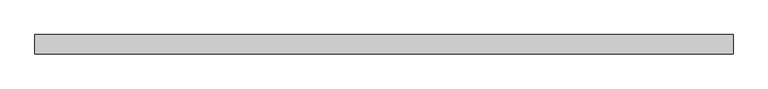
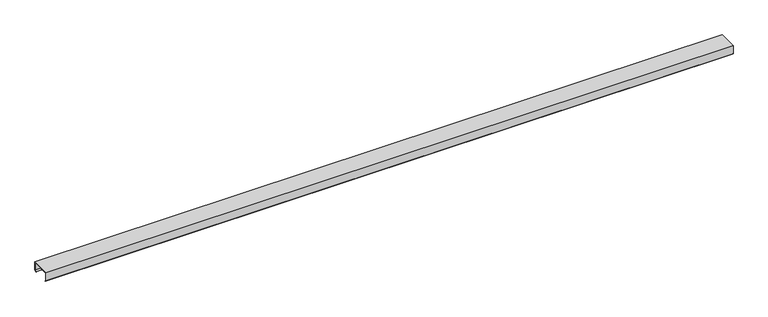
"""IFC4 building model written with IfcOpenShell, lengths in millimetres: proxy geometry, Generic Models 7:Generic Models 1:1:Generic Models 1:1 : Generic Models 7:Generic Models 1:337419:23 : Generic Models 7:Generic Models 1:1:Generic Models 1:1 : Generic Models 7:Generic Models 1:337419:306201."""

from ifc_helpers import new_model, si_unit, frame, origin, place, context, project, spatial, polyline, outline, extrude, source, transform, mapped, element, save


def generic_models_50360223(model_context):
    return source(origin(), model_context, "Body", "SweptSolid", [
        extrude(outline(polyline([(-578797.4913841, 4985.940625), (-578797.4913841, 4897.040625), (-578812.0845307, 4884.7955211), (-578813.870275, 4886.9236883), (-578800.2695091, 4898.336086), (-578800.2695091, 4983.1625), (-578997.9132591, 4983.1625), (-578997.9132591, 4898.336086), (-578984.3124931, 4886.9236883), (-578986.0982374, 4884.7955211), (-579000.6913841, 4897.040625), (-579000.6913841, 4985.940625), (-578797.4913841, 4985.940625)])), frame((560556.1617239, 0.0, 0.0), z_axis=(1.0, 0.0, 0.0), x_axis=(0.0, 1.0, 0.0)), (0.0, 0.0, 1.0), 7302.5),
    ])


if __name__ == "__main__":
    model = new_model("IFC4")
    model_context = context("Model", 3, world=origin())
    ifc_project = project(units=[si_unit("LENGTHUNIT", "METRE", prefix="MILLI")], contexts=[model_context])
    site = spatial("IfcSite", under=ifc_project)
    building = spatial("IfcBuilding", under=site)
    placement = place(None, origin())
    generic_models_shape = generic_models_50360223(model_context)
    element("IfcBuildingElementProxy", 1, Name="Generic Models 7:Generic Models 1:1:Generic Models 1:1 : Generic Models 7:Generic Models 1:337419:23 : Generic Models 7:Generic Models 1:1:Generic Models 1:1 : Generic Models 7:Generic Models 1:337419:306201", ObjectType="Generic Models 7:Generic Models 1:1:Generic Models 1:1 : Generic Models 7:Generic Models 1:337419:23 : Generic Models 7:Generic Models 1:1:Generic Models 1:1 : Generic Models 7:Generic Models 1:337419:306201", at=placement, inside=building, context=model_context, shape_type="MappedRepresentation", body=[
        mapped(generic_models_shape, transform((0.0, 0.0, 0.0), x_axis=(1.0, 0.0, 0.0), y_axis=(0.0, 1.0, 0.0), z_axis=(0.0, 0.0, 1.0))),
    ])
    save(model, "model.ifc")

# Revit data of these elements
# Type "Generic Models 7:Generic Models 1:1:Generic Models 1:1 : Generic Models 7:Generic Models 1:337419:23 : Generic Models 7:Generic Models 1:1:Generic Models 1:1 : Generic Models 7:Generic Models 1:337419:306201"
#   NameOverride = "Generic Models 7:Generic Models 1:1:Generic Models 1:1 : Generic Models 7:Generic Models 1:337419:306201"
#   ObjectTypeOverride = "Generic Models 1:1 : Generic Models 7:Generic Models 1:337419"
#   Reference = "Generic Models 1"
#   Tag = "306201"
# Element 1 (IfcBuildingElementProxy, "Generic Models 7:Generic Models 1:1:Generic Models 1:1 : Generic Models 7:Generic Models 1:337419:23 : Generic Models 7:Generic Models 1:1:Generic Models 1:1 : Generic Models 7:Generic Models 1:337419:306201")
#   Materials on its faces: "'ZEE' SECTION (8.0x3.5Z - SEE STRUCT. DWGS)"
# Materials
#   "'ZEE' SECTION (8.0x3.5Z - SEE STRUCT. DWGS)": class "Unassigned", colour RGB 210 209 208, transparency 0, Keynote = "M05121300.02", Cost = 0
